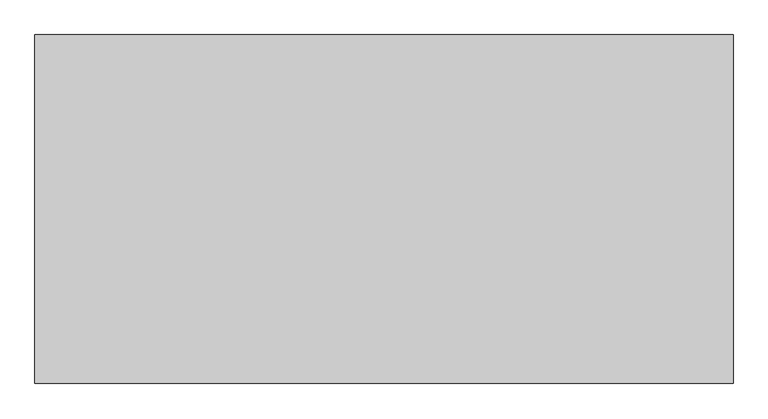
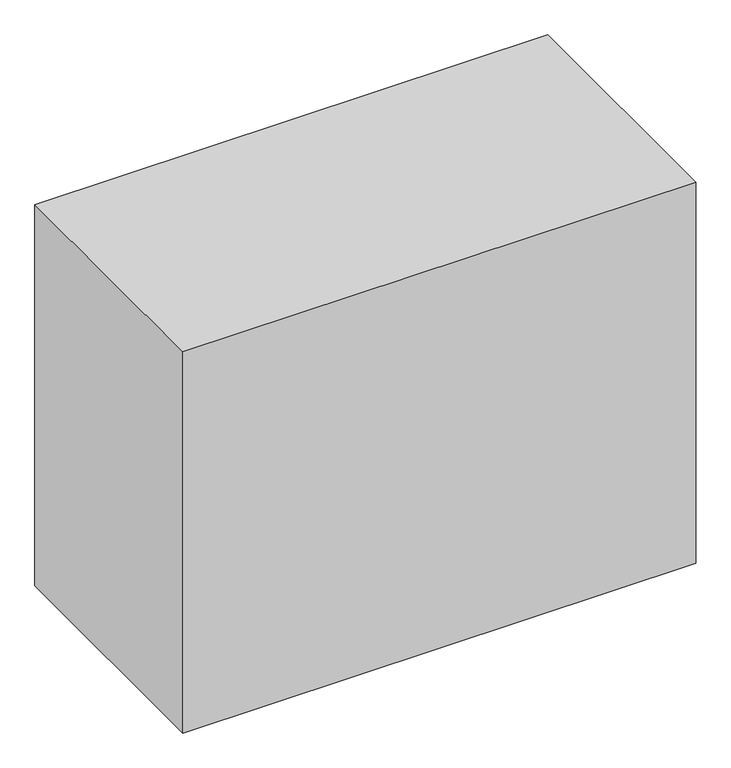
"""IFC4 building model written with IfcOpenShell, lengths in millimetres: proxy geometry, Space Planning Box_hec : Space Planning Box_hec."""

from ifc_helpers import new_model, si_unit, origin, origin_with_axes, place, context, project, spatial, polyline, outline, extrude, source, transform, mapped, element, save


def generic_models_85ff21bb(model_context):
    return source(origin(), model_context, "Body", "SweptSolid", [
        extrude(outline(polyline([(3500.0, 1750.0), (3500.0, -1750.0), (-3500.0, -1750.0), (-3500.0, 1750.0), (3500.0, 1750.0)])), origin_with_axes(), (0.0, 0.0, 1.0), 5500.0),
    ])


if __name__ == "__main__":
    model = new_model("IFC4")
    model_context = context("Model", 3, world=origin())
    ifc_project = project(units=[si_unit("LENGTHUNIT", "METRE", prefix="MILLI")], contexts=[model_context])
    site = spatial("IfcSite", under=ifc_project)
    building = spatial("IfcBuilding", under=site)
    placement = place(None, origin())
    generic_models_shape = generic_models_85ff21bb(model_context)
    element("IfcBuildingElementProxy", 1, Name="Space Planning Box_hec : Space Planning Box_hec", ObjectType="Space Planning Box_hec : Space Planning Box_hec", at=placement, inside=building, context=model_context, shape_type="MappedRepresentation", body=[
        mapped(generic_models_shape, transform((0.0, 0.0, 0.0), x_axis=(1.0, 0.0, 0.0), y_axis=(0.0, 1.0, 0.0), z_axis=(0.0, 0.0, 1.0))),
    ])
    save(model, "model.ifc")

# Revit data of these elements
# Type "Space Planning Box_hec : Space Planning Box_hec"
#   Type Comments = "..."
#   Room Name [instance default] = "?"
#   Interior Finish [instance default] = ""
#   Exterior Finish [instance default] = ""
#   Department [instance default] = ""
#   Assembly Code = "..."
#   ceiling height [instance default] = 0
#   Width [instance default] = 1524 mm
#   Program Area [instance default] = 0.00 m²
#   Length [instance default] = 1524 mm
#   Height [instance default] = 1524 mm
#   Area [instance default] = 2.32258 m²
#   Fill Color [instance default] = Cyan
#   Default Elevation = 0
# Element 1 (IfcBuildingElementProxy, "Space Planning Box_hec : Space Planning Box_hec")
#   Room Name = "Computer Room"
#   Exterior Finish = "N/A..N/A,,EW2..N/A..N/A"
#   Department = "AR"
#   Width = 7000 mm
#   Program Area = 24.50 m²
#   Length = 3500 mm
#   Height = 5500 mm
#   Area = 24.50 m²
#   Materials on its faces: "Cyan"
# Materials
#   "Cyan": class "Generic", colour RGB 0 255 255, transparency 0.2, Cost = 0
